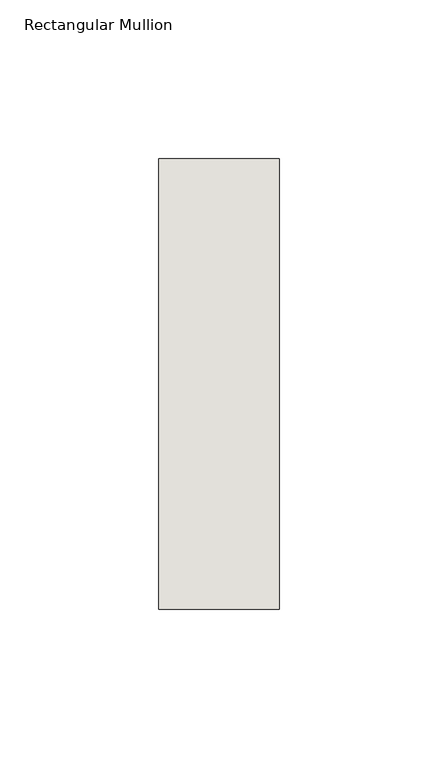
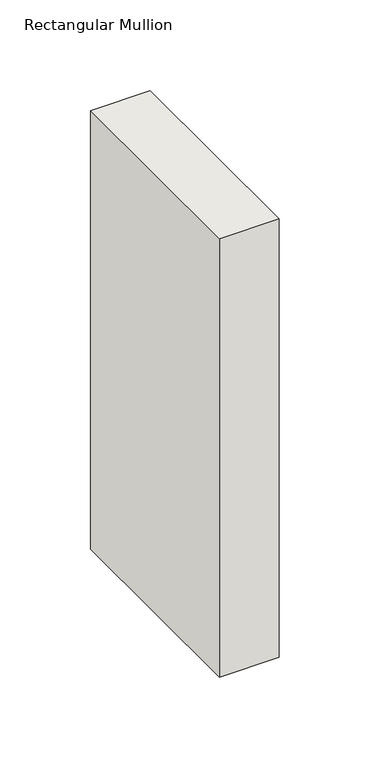
"""IFC4 building model written with IfcOpenShell, lengths in millimetres: wall geometry, Rectangular Mullion : NLRS_21_CWM_hsb-regel 38x142_gen_rsf."""

from ifc_helpers import new_model, si_unit, frame, origin, place, context, project, spatial, polyline, outline, extrude, source, transform, mapped, element, save


def rectangular_mullion_c53917db(model_context):
    return source(origin(), model_context, "Body", "SweptSolid", [
        extrude(outline(polyline([(19.0, -71.0), (-19.0, -71.0), (-19.0, 71.0), (19.0, 71.0), (19.0, -71.0)])), frame((0.0, 0.0, -295.0), z_axis=(0.0, 0.0, 1.0), x_axis=(1.0, 0.0, 0.0)), (0.0, 0.0, 1.0), 295.0),
    ])


if __name__ == "__main__":
    model = new_model("IFC4")
    model_context = context("Model", 3, world=origin())
    ifc_project = project(units=[si_unit("LENGTHUNIT", "METRE", prefix="MILLI")], contexts=[model_context])
    site = spatial("IfcSite", under=ifc_project)
    building = spatial("IfcBuilding", under=site)
    placement = place(None, origin())
    rectangular_mullion_shape = rectangular_mullion_c53917db(model_context)
    element("IfcWall", 1, ObjectType="Rectangular Mullion : NLRS_21_CWM_hsb-regel 38x142_gen_rsf", at=placement, inside=building, context=model_context, shape_type="MappedRepresentation", body=[
        mapped(rectangular_mullion_shape, transform((0.0, 0.0, 0.0), x_axis=(1.0, 0.0, 0.0), y_axis=(0.0, 1.0, 0.0), z_axis=(0.0, 0.0, 1.0))),
    ])
    save(model, "model.ifc")

# Revit data of these elements
# Type "Rectangular Mullion : NLRS_21_CWM_hsb-regel 38x142_gen_rsf"
#   Type IfcGUID = "07M7mRoiH1CR8m_RSKIwpF"
#   Assembly Code = "21.10"
#   IfcExportAs = "IfcWall"
#   built-in parameter 1007322 = 0.465879 (stored number, unit not read)
#   built-in parameter 1007321 = 0.062336 (stored number, unit not read)
#   built-in parameter 1007320 = 0.062336 (stored number, unit not read)
# Element 1 (IfcWall, "Rectangular Mullion : NLRS_21_CWM_hsb-regel 38x142_gen_rsf")
#   Materials on its faces: "NLRS_i2_hout naaldhout vuren_gen_rsf"
# Materials
#   "NLRS_i2_hout naaldhout vuren_gen_rsf": class "I - Hout", colour RGB 234 199 147, transparency 0, Keynote = "i2", Manufacturer = "Revit Standards Foundation", URL = "www.revitstandards.org", Description = "hout vuren", Cost = 0
